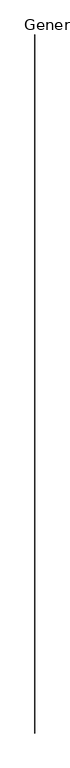
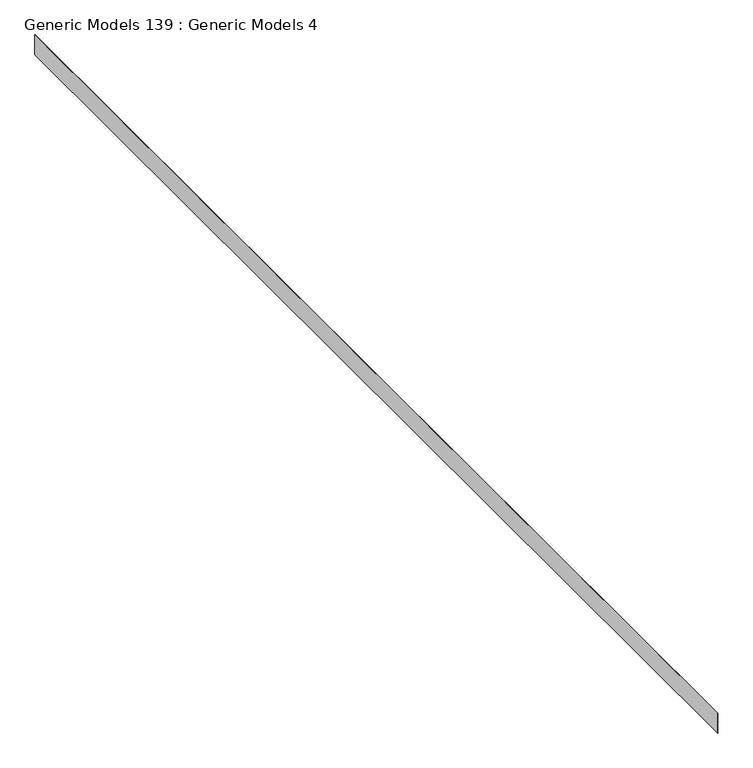
"""IFC4 building model written with IfcOpenShell, lengths in millimetres: proxy geometry, Generic Models 139 : Generic Models 4."""

import ifcopenshell
import ifcopenshell.guid

model = None  # the IFC model being written
_history = None  # IfcOwnerHistory: only IFC2X3 demands one
_inside = {}  # id of a spatial element -> (the spatial element, [elements in it])
_under = {}  # id of a project, library or spatial element -> (it, [spatial elements below it])
_declared = {}  # id of a project -> (the project, [libraries it declares])
_typed = {}  # id of a type object -> (the type object, [elements of that type])
_made_of = {}  # id of a material, layer set ... -> (it, [elements and type objects made of it])


def new_model(schema):
    """Start an empty IFC model of exactly this schema.

    Asked for "IFC4X3", IfcOpenShell would pick the latest addendum, in which some entities
    have other attributes; the version numbers below select the first issue.
    IFC2X3 requires an IfcOwnerHistory on every rooted entity: one is made here for all.
    """
    global model, _history
    if schema == "IFC4X3":
        model = ifcopenshell.file(schema_version=(4, 3, 0, 0))
    else:
        model = ifcopenshell.file(schema=schema)
    _inside.clear()
    _under.clear()
    _declared.clear()
    _typed.clear()
    _made_of.clear()
    _history = None
    if model.schema == "IFC2X3":
        org = make("IfcOrganization", Name="unknown")
        user = make(
            "IfcPersonAndOrganization",
            ThePerson=make("IfcPerson", FamilyName="unknown"),
            TheOrganization=org,
        )
        app = make(
            "IfcApplication",
            ApplicationDeveloper=org,
            Version="unknown",
            ApplicationFullName="unknown",
            ApplicationIdentifier="unknown",
        )
        _history = make(
            "IfcOwnerHistory",
            OwningUser=user,
            OwningApplication=app,
            ChangeAction="ADDED",
            CreationDate=0,
        )
    return model


def make(cls, **values):
    """One entity of the class cls with the attributes given. An attribute that is None is left unset."""
    return model.create_entity(
        cls, **{name: value for name, value in values.items() if value is not None}
    )


def rooted(cls, **values):
    """An entity with a GlobalId (a new one), such as an element, a storey or a relation."""
    return make(cls, GlobalId=ifcopenshell.guid.new(), OwnerHistory=_history, **values)


def si_unit(unit_type, name, prefix=None):
    """IfcSIUnit, for example si_unit("LENGTHUNIT", "METRE", prefix="MILLI")."""
    return make("IfcSIUnit", UnitType=unit_type, Prefix=prefix, Name=name)


def assignment(units):
    """IfcUnitAssignment: the units of a project."""
    return None if units is None else make("IfcUnitAssignment", Units=units)


def point(xyz):
    """IfcCartesianPoint."""
    return None if xyz is None else make("IfcCartesianPoint", Coordinates=xyz)


def direction(xyz):
    """IfcDirection."""
    return None if xyz is None else make("IfcDirection", DirectionRatios=xyz)


def frame(location, z_axis=None, x_axis=None):
    """IfcAxis2Placement3D, a coordinate frame: its origin and axes. An axis left out is left unset."""
    return make(
        "IfcAxis2Placement3D",
        Location=point(location),
        Axis=direction(z_axis),
        RefDirection=direction(x_axis),
    )


def origin():
    """The frame at (0, 0, 0) with its axes left unset."""
    return frame((0.0, 0.0, 0.0))


def place(relative_to, where):
    """IfcLocalPlacement: puts the frame where relative to a parent placement (None: the world)."""
    return make(
        "IfcLocalPlacement", PlacementRelTo=relative_to, RelativePlacement=where
    )


def context(
    kind, dimensions, precision=None, world=None, true_north=None, identifier=None
):
    """IfcGeometricRepresentationContext, for example the 3D "Model" context."""
    return make(
        "IfcGeometricRepresentationContext",
        ContextIdentifier=identifier,
        ContextType=kind,
        CoordinateSpaceDimension=dimensions,
        Precision=precision,
        WorldCoordinateSystem=world,
        TrueNorth=true_north,
    )


def project(units=None, contexts=None):
    """IfcProject with its units and contexts."""
    return rooted(
        "IfcProject",
        Name="project",
        RepresentationContexts=contexts,
        UnitsInContext=assignment(units),
    )


def spatial(cls, under=None, at=None, **own):
    """A site, building, storey or space (cls), placed at a placement, below another one or the project."""
    s = rooted(cls, ObjectPlacement=at, **own)
    if under is not None:
        _under.setdefault(under.id(), (under, []))[1].append(s)
    return s


def polyline(points):
    """IfcPolyline through the points."""
    return make("IfcPolyline", Points=[point(p) for p in points])


def outline(outer, holes=None, kind="AREA"):
    """IfcArbitraryClosedProfileDef: a profile drawn as a closed curve; with holes, ...WithVoids."""
    if holes is None:
        return make("IfcArbitraryClosedProfileDef", ProfileType=kind, OuterCurve=outer)
    return make(
        "IfcArbitraryProfileDefWithVoids",
        ProfileType=kind,
        OuterCurve=outer,
        InnerCurves=holes,
    )


def extrude(swept, where, along, depth):
    """IfcExtrudedAreaSolid: the profile swept, set in the frame where, extruded along a direction by depth."""
    return make(
        "IfcExtrudedAreaSolid",
        SweptArea=swept,
        Position=where,
        ExtrudedDirection=direction(along),
        Depth=depth,
    )


def shape(context_of_items, identifier, shape_type, items):
    """IfcShapeRepresentation: the items that make up one representation, for example the "Body"."""
    return make(
        "IfcShapeRepresentation",
        ContextOfItems=context_of_items,
        RepresentationIdentifier=identifier,
        RepresentationType=shape_type,
        Items=items,
    )


def source(mapping_origin, context_of_items, identifier, shape_type, items):
    """IfcRepresentationMap: a shape defined once, which mapped items show again and again."""
    return make(
        "IfcRepresentationMap",
        MappingOrigin=mapping_origin,
        MappedRepresentation=shape(context_of_items, identifier, shape_type, items),
    )


def transform(
    local_origin,
    x_axis=None,
    y_axis=None,
    z_axis=None,
    scale=None,
    scale2=None,
    scale3=None,
    uniform=True,
):
    """IfcCartesianTransformationOperator3D, or its non-uniform kind. x_axis, y_axis, z_axis: its Axis1, 2, 3."""
    if uniform:
        return make(
            "IfcCartesianTransformationOperator3D",
            Axis1=direction(x_axis),
            Axis2=direction(y_axis),
            LocalOrigin=point(local_origin),
            Scale=scale,
            Axis3=direction(z_axis),
        )
    return make(
        "IfcCartesianTransformationOperator3DnonUniform",
        Axis1=direction(x_axis),
        Axis2=direction(y_axis),
        LocalOrigin=point(local_origin),
        Scale=scale,
        Axis3=direction(z_axis),
        Scale2=scale2,
        Scale3=scale3,
    )


def mapped(mapping_source, mapping_target):
    """IfcMappedItem: shows the shape of a source again, moved by a transform."""
    return make(
        "IfcMappedItem", MappingSource=mapping_source, MappingTarget=mapping_target
    )


def made_of(thing, what):
    """Note that an element or type object is made of a material, layer set ...; save() writes the relation."""
    if what is not None:
        _made_of.setdefault(what.id(), (what, []))[1].append(thing)
    return thing


def element(
    cls,
    number,
    at=None,
    inside=None,
    cuts=None,
    type_object=None,
    material=None,
    context=None,
    identifier="Body",
    shape_type=None,
    held_by="IfcProductDefinitionShape",
    body=None,
    shapes=None,
    **own,
):
    """One element of the class cls, such as IfcWall. Its Tag is "e" and its number.

    at: its placement. inside: the storey or other place that contains it. cuts: it is an
    opening in that element (IfcRelVoidsElement). A single representation is given by context,
    identifier, shape_type and body (its items); several are given by shapes. held_by: the class
    of the entity that holds the representations. save() writes the other relations.
    """
    e = rooted(cls, Tag="e%d" % number, ObjectPlacement=at, **own)
    if body is not None:
        shapes = [shape(context, identifier, shape_type, body)]
    if shapes is not None:
        e.Representation = make(held_by, Representations=shapes)
    if inside is not None:
        _inside.setdefault(inside.id(), (inside, []))[1].append(e)
    if cuts is not None:
        rooted(
            "IfcRelVoidsElement", RelatingBuildingElement=cuts, RelatedOpeningElement=e
        )
    if type_object is not None:
        _typed.setdefault(type_object.id(), (type_object, []))[1].append(e)
    return made_of(e, material)


def aggregate(whole, parts):
    """IfcRelAggregates: a whole, such as a stair, and the parts it consists of."""
    return rooted("IfcRelAggregates", RelatingObject=whole, RelatedObjects=parts)


def save(model, path):
    """Write the relations noted so far, then the file.

    IfcRelAggregates (storeys below a building ...), IfcRelContainedInSpatialStructure (elements
    in a storey), IfcRelDefinesByType, IfcRelAssociatesMaterial and IfcRelDeclares: one each for
    every whole, place, type object, material and project.
    """
    for whole, parts in _under.values():
        aggregate(whole, parts)
    for where, things in _inside.values():
        rooted(
            "IfcRelContainedInSpatialStructure",
            RelatedElements=things,
            RelatingStructure=where,
        )
    for kind, things in _typed.values():
        rooted("IfcRelDefinesByType", RelatedObjects=things, RelatingType=kind)
    for what, things in _made_of.values():
        rooted("IfcRelAssociatesMaterial", RelatedObjects=things, RelatingMaterial=what)
    for by, libraries in _declared.values():
        rooted("IfcRelDeclares", RelatingContext=by, RelatedDefinitions=libraries)
    model.write(path)


def generic_models_139_generic_models_4_d797433e(model_context):
    return source(origin(), model_context, "Body", "SweptSolid", [
        extrude(outline(polyline([(-10231.3472239, -5493.3230338), (-10232.9347239, -5493.3230338), (-10232.9347239, 7054.2769662), (-10231.3472239, 7054.2769662), (-10231.3472239, -5493.3230338)])), frame((0.0, 0.0, 122573.1444509), z_axis=(0.0, 0.0, 1.0), x_axis=(1.0, 0.0, 0.0)), (0.0, 0.0, 1.0), 220.5790364),
    ])


if __name__ == "__main__":
    model = new_model("IFC4")
    model_context = context("Model", 3, world=origin())
    ifc_project = project(units=[si_unit("LENGTHUNIT", "METRE", prefix="MILLI")], contexts=[model_context])
    site = spatial("IfcSite", under=ifc_project)
    building = spatial("IfcBuilding", under=site)
    placement = place(None, origin())
    generic_models_139_generic_models_4_shape = generic_models_139_generic_models_4_d797433e(model_context)
    element("IfcBuildingElementProxy", 1, Name="Generic Models 139 : Generic Models 4", ObjectType="Generic Models 139 : Generic Models 4", at=placement, inside=building, context=model_context, shape_type="MappedRepresentation", body=[
        mapped(generic_models_139_generic_models_4_shape, transform((0.0, 0.0, 0.0), x_axis=(1.0, 0.0, 0.0), y_axis=(0.0, 1.0, 0.0), z_axis=(0.0, 0.0, 1.0))),
    ])
    save(model, "model.ifc")

# Revit data of these elements
# Element 1 (IfcBuildingElementProxy, "Generic Models 139 : Generic Models 4")
#   Materials on its faces: "_WIRE LATH"
# Materials
#   "_WIRE LATH": class "Generic", colour RGB 73 45 73, transparency 0, Cost = 0
